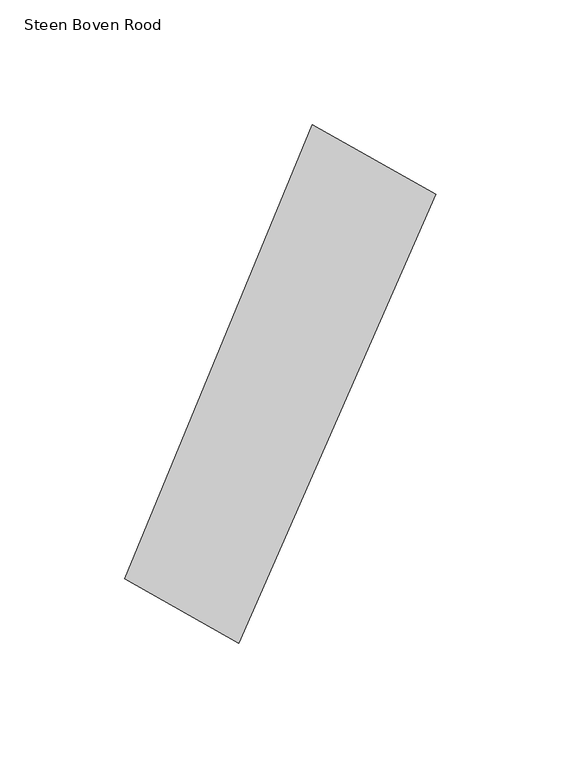
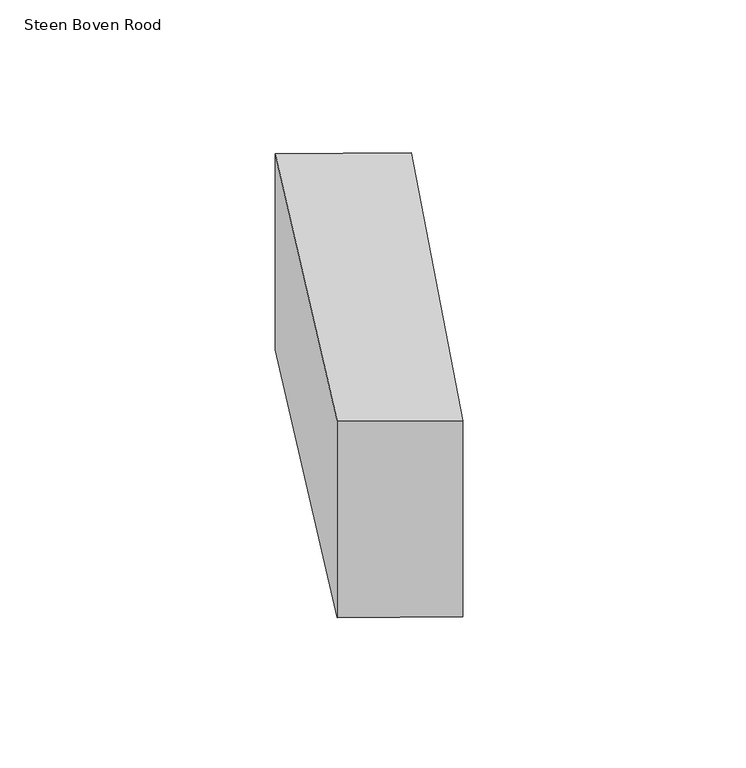
"""IFC4 building model written with IfcOpenShell, lengths in millimetres: proxy geometry, 00_GMA_steen_versie_4 : Steen Boven Rood."""

from ifc_helpers import new_model, si_unit, origin, origin_with_axes, place, context, project, spatial, polyline, outline, extrude, source, transform, mapped, element, save


def steen_boven_rood_14afb36a(model_context):
    return source(origin(), model_context, "Body", "SweptSolid", [
        extrude(outline(polyline([(141.5862146, 163.0770734), (62.8174194, -16.3968271), (17.22364, 9.2892089), (92.2206462, 190.9006564), (141.5862146, 163.0770734)])), origin_with_axes(), (0.0, 0.0, 1.0), 100.0),
    ])


if __name__ == "__main__":
    model = new_model("IFC4")
    model_context = context("Model", 3, world=origin())
    ifc_project = project(units=[si_unit("LENGTHUNIT", "METRE", prefix="MILLI")], contexts=[model_context])
    site = spatial("IfcSite", under=ifc_project)
    building = spatial("IfcBuilding", under=site)
    placement = place(None, origin())
    steen_boven_rood_shape = steen_boven_rood_14afb36a(model_context)
    element("IfcBuildingElementProxy", 1, Name="00_GMA_steen_versie_4 : Steen Boven Rood", ObjectType="00_GMA_steen_versie_4 : Steen Boven Rood", at=placement, inside=building, context=model_context, shape_type="MappedRepresentation", body=[
        mapped(steen_boven_rood_shape, transform((0.0, 0.0, 0.0), x_axis=(1.0, 0.0, 0.0), y_axis=(0.0, 1.0, 0.0), z_axis=(0.0, 0.0, 1.0))),
    ])
    save(model, "model.ifc")

# Revit data of these elements
# Type "00_GMA_steen_versie_4 : Steen Boven Rood"
#   StootVoegHalfBoven [instance default] = 5 mm
#   StootVoegHalf [instance default] = 5 mm
#   StootVoegBreedteOnder = 10 mm
#   StootVoegBreedteBoven = 10 mm
#   Steendikte = 100 mm
#   LintVoegOnderHalf = 5 mm
#   LintVoegOnder = 10 mm
#   LintVoegBovenHalf = 0 mm
#   LintVoegBoven = 0 mm
#   materiaal = 21_steen_rood
#   MateriaalVoeg = none
#   Default Elevation = 0
# Element 1 (IfcBuildingElementProxy, "00_GMA_steen_versie_4 : Steen Boven Rood")
#   Materials on its faces: "21_steen_rood"
# Materials
#   "21_steen_rood": class "Unassigned", colour RGB 213 111 43, transparency 0, Cost = 0
